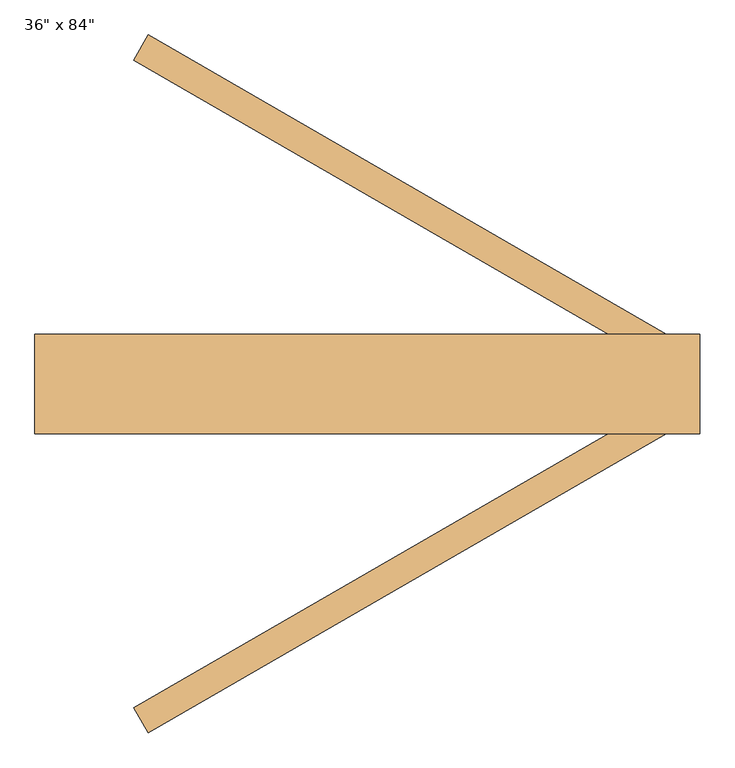
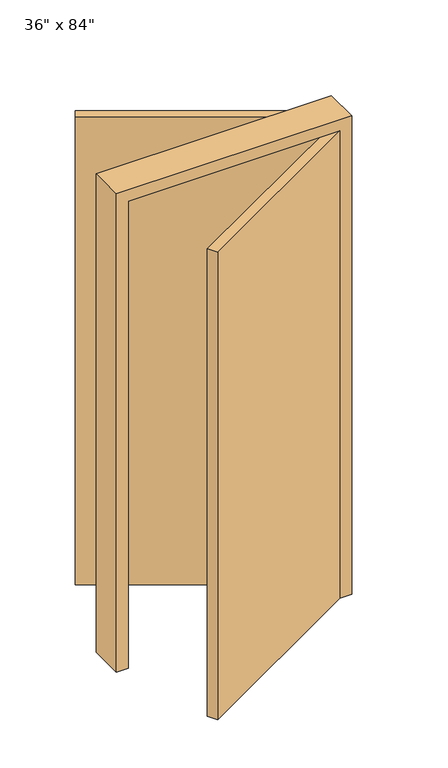
"""IFC4 building model written with IfcOpenShell, lengths in millimetres: door geometry."""

from ifc_helpers import new_model, si_unit, frame, origin, origin_with_axes, place, context, project, spatial, polyline, outline, extrude, source, transform, mapped, element, save


def door_c5e3a2c4(model_context):
    return source(origin(), model_context, "Body", "SweptSolid", [
        extrude(outline(polyline([(-356.9186292, -494.3958963), (434.975, -37.1958963), (457.2, -75.6907255), (-334.6936292, -532.8907255), (-356.9186292, -494.3958963)])), origin_with_axes(), (0.0, 0.0, 1.0), 2133.6),
        extrude(outline(polyline([(-356.9186292, 495.4144453), (-334.6936292, 533.9092745), (457.2, 76.7092745), (434.975, 38.2144453), (-356.9186292, 495.4144453)])), origin_with_axes(), (0.0, 0.0, 1.0), 2133.6),
        extrude(outline(polyline([(0.0, 457.2), (0.0, 508.0), (2184.4, 508.0), (2184.4, -508.0), (0.0, -508.0), (0.0, -457.2), (2133.6, -457.2), (2133.6, 457.2), (0.0, 457.2)])), frame((0.0, -75.6907255, 0.0), z_axis=(0.0, 1.0, 0.0), x_axis=(0.0, 0.0, 1.0)), (0.0, 0.0, 1.0), 152.4),
    ])


if __name__ == "__main__":
    model = new_model("IFC4")
    model_context = context("Model", 3, world=origin())
    ifc_project = project(units=[si_unit("LENGTHUNIT", "METRE", prefix="MILLI")], contexts=[model_context])
    site = spatial("IfcSite", under=ifc_project)
    building = spatial("IfcBuilding", under=site)
    placement = place(None, origin())
    door_shape = door_c5e3a2c4(model_context)
    element("IfcDoor", 1, ObjectType="Communicating Door : 36\" x 84\"", at=placement, inside=building, context=model_context, shape_type="MappedRepresentation", body=[
        mapped(door_shape, transform((0.0, 0.0, 0.0), x_axis=(1.0, 0.0, 0.0), y_axis=(0.0, 1.0, 0.0), z_axis=(0.0, 0.0, 1.0))),
    ])
    save(model, "model.ifc")

# Revit data of these elements
# Type "Communicating Door : 36\" x 84\""
#   Type Mark = "31"
#   Thickness = 0' - 1 3/4"
#   Swing Angle [instance default] = 30.00°
#   Rough Width [instance default] = 3' - 4"
#   Rough Height [instance default] = 7' - 2"
#   Frame Width [instance default] = 0' - 2"
#   Height = 7' - 0"
#   Width = 3' - 0"
#   Frame Offset [instance default] = 0' - 1"
#   Frame Head [instance default] = 0' - 2"
#   Frame Depth [instance default] = 0' - 6"
#   Function = 0
#   Wall Closure = 3
#   Frame Material = none
#   Door Material = none
